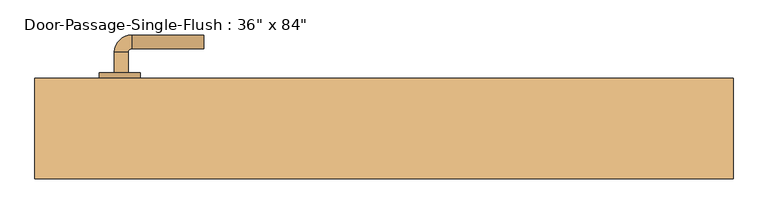
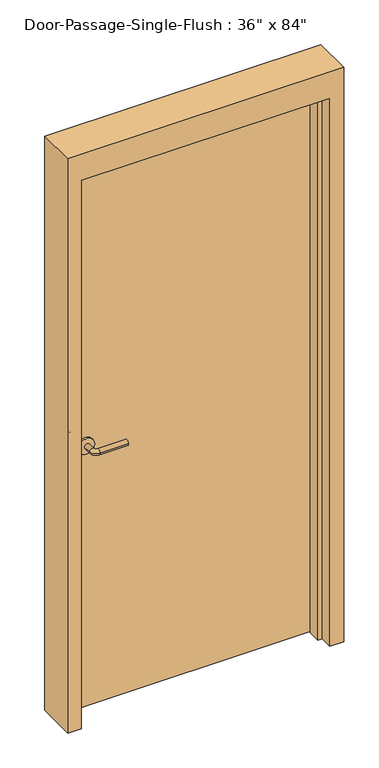
"""IFC4 building model written with IfcOpenShell, lengths in millimetres: door geometry."""

from ifc_helpers import new_model, si_unit, point, frame, frame_2d, origin, origin_with_axes, place, context, project, spatial, polyline, circle_curve, ellipse_curve, trimmed, segment, composite_curve, outline, extrude, faceted_brep, source, transform, mapped, element, save
from ifc_brep_helpers import plane_surface, cylinder_surface, revolved_surface, advanced_brep


def door_a255baf1(model_context):
    return source(origin(), model_context, "Body", "SolidModel", [
        advanced_brep(
        [(-392.190625, -1.65, 1016.0), (-372.190625, -1.65, 1016.0), (-372.190625, -31.65, 1016.0), (-392.190625, -31.65, 1016.0), (-367.190625, -36.65, 1016.0), (-367.190625, -56.65, 1016.0), (-262.190625, -56.65, 1016.0), (-262.190625, -36.65, 1016.0)],
        [
            (0, 1, circle_curve(frame((-382.190625, -1.65, 1016.0), z_axis=(0.0, 1.0, 0.0), x_axis=(1.0, 0.0, 0.0)), 10.0)),
            (1, 0, circle_curve(frame((-382.190625, -1.65, 1016.0), z_axis=(0.0, 1.0, 0.0), x_axis=(1.0, 0.0, 0.0)), 10.0)),
            (1, 2),
            (2, 3, circle_curve(frame((-382.190625, -31.65, 1016.0), z_axis=(0.0, 1.0, 0.0), x_axis=(1.0, 0.0, 0.0)), 10.0)),
            (3, 0),
            (3, 2, circle_curve(frame((-382.190625, -31.65, 1016.0), z_axis=(0.0, 1.0, 0.0), x_axis=(1.0, 0.0, 0.0)), 10.0)),
            (4, 5, circle_curve(frame((-367.190625, -46.65, 1016.0), z_axis=(-1.0, 0.0, 0.0), x_axis=(0.0, 1.0, 0.0)), 10.0)),
            (5, 3, circle_curve(frame((-367.190625, -31.65, 1016.0), z_axis=(0.0, 0.0, -1.0), x_axis=(-1.0, 0.0, 0.0)), 25.0)),
            (2, 4, circle_curve(frame((-367.190625, -31.65, 1016.0), z_axis=(0.0, 0.0, 1.0), x_axis=(-1.0, 0.0, 0.0)), 5.0)),
            (5, 4, circle_curve(frame((-367.190625, -46.65, 1016.0), z_axis=(-1.0, 0.0, 0.0), x_axis=(0.0, 1.0, 0.0)), 10.0)),
            (6, 7, circle_curve(frame((-262.190625, -46.65, 1016.0), z_axis=(1.0, 0.0, 0.0), x_axis=(0.0, 1.0, 0.0)), 10.0)),
            (7, 6, circle_curve(frame((-262.190625, -46.65, 1016.0), z_axis=(1.0, 0.0, 0.0), x_axis=(0.0, 1.0, 0.0)), 10.0)),
            (4, 7),
            (6, 5),
        ],
        [
            plane_surface(frame((-382.190625, -1.65, 1016.0), z_axis=(0.0, 1.0, 0.0), x_axis=(0.0, 0.0, 1.0))),
            cylinder_surface(frame((-382.190625, -1.65, 1016.0), z_axis=(0.0, 1.0, 0.0), x_axis=(1.0, 0.0, 0.0)), 10.0),
            revolved_surface(trimmed(ellipse_curve(frame((-382.190625, -31.65, 1016.0), z_axis=(0.0, -1.0, 0.0), x_axis=(1.0, 0.0, 0.0)), 10.0, 10.0), [point((-392.190625, -31.65, 1016.0))], [point((-372.190625, -31.65, 1016.0))], True, "CARTESIAN"), (-367.190625, -31.65, 1016.0), (0.0, 0.0, -1.0)),
            revolved_surface(trimmed(ellipse_curve(frame((-382.190625, -31.65, 1016.0), z_axis=(0.0, -1.0, 0.0), x_axis=(1.0, 0.0, 0.0)), 10.0, 10.0), [point((-372.190625, -31.65, 1016.0))], [point((-392.190625, -31.65, 1016.0))], True, "CARTESIAN"), (-367.190625, -31.65, 1016.0), (0.0, 0.0, -1.0)),
            plane_surface(frame((-262.190625, -46.65, 1016.0), z_axis=(1.0, 0.0, 0.0), x_axis=(0.0, 0.0, 1.0))),
            cylinder_surface(frame((-367.190625, -46.65, 1016.0), z_axis=(-1.0, 0.0, 0.0), x_axis=(0.0, 1.0, 0.0)), 10.0),
        ],
        [
            (0, [[1, 2]]),
            (1, [[3, 4, 5, -2]]),
            (1, [[-5, 6, -3, -1]]),
            (2, [[7, 8, -4, 9]]),
            (3, [[10, -9, -6, -8]]),
            (4, [[11, 12]]),
            (5, [[13, -11, 14, -7]]),
            (5, [[-14, -12, -13, -10]]),
        ],
    ),
        extrude(outline(composite_curve([segment(trimmed(circle_curve(frame_2d((1016.0, -384.690625)), 30.0), [point((1016.0, -414.690625))], [point((1016.0, -354.690625))], False, "CARTESIAN"), True, "CONTINUOUS"), segment(trimmed(circle_curve(frame_2d((1016.0, -384.690625)), 30.0), [point((1016.0, -354.690625))], [point((1016.0, -414.690625))], False, "CARTESIAN"), True, "CONTINUOUS")], self_intersect=False)), frame((0.0, -1.65, 0.0), z_axis=(0.0, 1.0, 0.0), x_axis=(0.0, 0.0, 1.0)), (0.0, 0.0, 1.0), 8.0),
        advanced_brep(
        [(-392.190625, 58.8, 1016.0), (-372.190625, 58.8, 1016.0), (-392.190625, 88.8, 1016.0), (-372.190625, 88.8, 1016.0), (-367.190625, 93.8, 1016.0), (-367.190625, 113.8, 1016.0), (-262.190625, 113.8, 1016.0), (-262.190625, 93.8, 1016.0)],
        [
            (0, 1, circle_curve(frame((-382.190625, 58.8, 1016.0), z_axis=(0.0, -1.0, 0.0), x_axis=(1.0, 0.0, 0.0)), 10.0)),
            (1, 0, circle_curve(frame((-382.190625, 58.8, 1016.0), z_axis=(0.0, -1.0, 0.0), x_axis=(1.0, 0.0, 0.0)), 10.0)),
            (0, 2),
            (2, 3, circle_curve(frame((-382.190625, 88.8, 1016.0), z_axis=(0.0, -1.0, 0.0), x_axis=(1.0, 0.0, 0.0)), 10.0)),
            (3, 1),
            (3, 2, circle_curve(frame((-382.190625, 88.8, 1016.0), z_axis=(0.0, -1.0, 0.0), x_axis=(1.0, 0.0, 0.0)), 10.0)),
            (4, 3, circle_curve(frame((-367.190625, 88.8, 1016.0), z_axis=(0.0, 0.0, 1.0), x_axis=(-1.0, 0.0, 0.0)), 5.0)),
            (2, 5, circle_curve(frame((-367.190625, 88.8, 1016.0), z_axis=(0.0, 0.0, -1.0), x_axis=(-1.0, 0.0, 0.0)), 25.0)),
            (5, 4, circle_curve(frame((-367.190625, 103.8, 1016.0), z_axis=(-1.0, 0.0, 0.0), x_axis=(0.0, -1.0, 0.0)), 10.0)),
            (4, 5, circle_curve(frame((-367.190625, 103.8, 1016.0), z_axis=(-1.0, 0.0, 0.0), x_axis=(0.0, -1.0, 0.0)), 10.0)),
            (6, 7, circle_curve(frame((-262.190625, 103.8, 1016.0), z_axis=(1.0, 0.0, 0.0), x_axis=(0.0, -1.0, 0.0)), 10.0)),
            (7, 6, circle_curve(frame((-262.190625, 103.8, 1016.0), z_axis=(1.0, 0.0, 0.0), x_axis=(0.0, -1.0, 0.0)), 10.0)),
            (5, 6),
            (7, 4),
        ],
        [
            plane_surface(frame((-382.190625, 58.8, 1016.0), z_axis=(0.0, -1.0, 0.0), x_axis=(0.0, 0.0, 1.0))),
            cylinder_surface(frame((-382.190625, 58.8, 1016.0), z_axis=(0.0, -1.0, 0.0), x_axis=(1.0, 0.0, 0.0)), 10.0),
            revolved_surface(trimmed(ellipse_curve(frame((-382.190625, 88.8, 1016.0), z_axis=(0.0, -1.0, 0.0), x_axis=(1.0, 0.0, 0.0)), 10.0, 10.0), [point((-392.190625, 88.8, 1016.0))], [point((-372.190625, 88.8, 1016.0))], True, "CARTESIAN"), (-367.190625, 88.8, 1016.0), (0.0, 0.0, -1.0)),
            revolved_surface(trimmed(ellipse_curve(frame((-382.190625, 88.8, 1016.0), z_axis=(0.0, -1.0, 0.0), x_axis=(1.0, 0.0, 0.0)), 10.0, 10.0), [point((-372.190625, 88.8, 1016.0))], [point((-392.190625, 88.8, 1016.0))], True, "CARTESIAN"), (-367.190625, 88.8, 1016.0), (0.0, 0.0, -1.0)),
            plane_surface(frame((-262.190625, 103.8, 1016.0), z_axis=(1.0, 0.0, 0.0), x_axis=(0.0, 0.0, 1.0))),
            cylinder_surface(frame((-367.190625, 103.8, 1016.0), z_axis=(-1.0, 0.0, 0.0), x_axis=(0.0, -1.0, 0.0)), 10.0),
        ],
        [
            (0, [[1, 2]]),
            (1, [[-1, 3, 4, 5]]),
            (1, [[-2, -5, 6, -3]]),
            (2, [[7, -4, 8, 9]]),
            (3, [[-8, -6, -7, 10]]),
            (4, [[11, 12]]),
            (5, [[-9, 13, -12, 14]]),
            (5, [[-10, -14, -11, -13]]),
        ],
    ),
        extrude(outline(composite_curve([segment(trimmed(circle_curve(frame_2d((1016.0, -384.690625)), 30.0), [point((1016.0, -414.690625))], [point((1016.0, -354.690625))], False, "CARTESIAN"), True, "CONTINUOUS"), segment(trimmed(circle_curve(frame_2d((1016.0, -384.690625)), 30.0), [point((1016.0, -354.690625))], [point((1016.0, -414.690625))], False, "CARTESIAN"), True, "CONTINUOUS")], self_intersect=False)), frame((0.0, 50.8, 0.0), z_axis=(0.0, 1.0, 0.0), x_axis=(0.0, 0.0, 1.0)), (0.0, 0.0, 1.0), 8.0),
        faceted_brep([(457.2, 1.5875, 0.0), (457.2, 50.8, 0.0), (508.0, 50.8, 0.0), (508.0, -95.25, 0.0), (457.2, -95.25, 0.0), (457.2, -46.0375, 0.0), (441.325, -46.0375, 0.0), (441.325, 1.5875, 0.0), (457.2, 1.5875, 2133.6), (457.2, 50.8, 2133.6), (-457.2, 50.8, 2133.6), (-457.2, 50.8, 0.0), (-508.0, 50.8, 0.0), (-508.0, 50.8, 2235.2), (508.0, 50.8, 2235.2), (508.0, -95.25, 2235.2), (-508.0, -95.25, 2235.2), (-508.0, -95.25, 0.0), (-457.2, -95.25, 0.0), (-457.2, -95.25, 2133.6), (457.2, -95.25, 2133.6), (457.2, -46.0375, 2133.6), (-457.2, -46.0375, 2133.6), (-457.2, -46.0375, 0.0), (-441.325, -46.0375, 0.0), (-441.325, -46.0375, 2117.725), (441.325, -46.0375, 2117.725), (441.325, 1.5875, 2117.725), (-441.325, 1.5875, 2117.725), (-441.325, 1.5875, 0.0), (-457.2, 1.5875, 0.0), (-457.2, 1.5875, 2133.6)], [[[0, 1, 2, 3, 4, 5, 6, 7]], [[1, 0, 8, 9]], [[2, 1, 9, 10, 11, 12, 13, 14]], [[3, 2, 14, 15]], [[4, 3, 15, 16, 17, 18, 19, 20]], [[5, 4, 20, 21]], [[6, 5, 21, 22, 23, 24, 25, 26]], [[7, 6, 26, 27]], [[0, 7, 27, 28, 29, 30, 31, 8]], [[9, 8, 31, 10]], [[20, 19, 22, 21]], [[26, 25, 28, 27]], [[12, 11, 30, 29, 24, 23, 18, 17]], [[11, 10, 31, 30]], [[13, 12, 17, 16]], [[19, 18, 23, 22]], [[25, 24, 29, 28]], [[15, 14, 13, 16]]]),
        extrude(outline(polyline([(457.2, 6.35), (-457.2, 6.35), (-457.2, 50.8), (457.2, 50.8), (457.2, 6.35)])), origin_with_axes(), (0.0, 0.0, 1.0), 2133.6),
    ])


if __name__ == "__main__":
    model = new_model("IFC4")
    model_context = context("Model", 3, world=origin())
    ifc_project = project(units=[si_unit("LENGTHUNIT", "METRE", prefix="MILLI")], contexts=[model_context])
    site = spatial("IfcSite", under=ifc_project)
    building = spatial("IfcBuilding", under=site)
    placement = place(None, origin())
    door_shape = door_a255baf1(model_context)
    element("IfcDoor", 1, ObjectType="Door-Passage-Single-Flush : 36\" x 84\"", at=placement, inside=building, context=model_context, shape_type="MappedRepresentation", body=[
        mapped(door_shape, transform((0.0, 0.0, 0.0), x_axis=(1.0, 0.0, 0.0), y_axis=(0.0, 1.0, 0.0), z_axis=(0.0, 0.0, 1.0))),
    ])
    save(model, "model.ifc")

# Revit data of these elements
# Type "Door-Passage-Single-Flush : 36\" x 84\""
#   Type Mark = "35"
#   Assembly Code = "B2030200"
#   Analytic Construction = "Wooden"
#   Thickness = 0' - 1 3/4"
#   Thermal Resistance (R) = 2.5876 (h·ft²·°F)/BTU
#   Swing Angle [instance default] = 90.00°
#   Strike Height = 3' - 4"
#   Rough Width [instance default] = 3' - 4"
#   Rough Height [instance default] = 7' - 4"
#   MF Opening Height [instance default] = 0' - 4"
#   MF Opening Width [instance default] = 0' - 4"
#   Inset Calculate [instance default] = 0' - 4"
#   Masonry Inset [instance default] = 0' - 1"
#   Height = 7' - 0"
#   Width = 3' - 0"
#   Heat Transfer Coefficient (U) = 0.3865 BTU/(h·ft²·°F)
#   Masonry Frame Depth = 0' - 5 3/4"
#   Masonry Frame [instance default] = yes
#   Function = 1
#   Dry Wall Frame [instance default] = no
#   Panel Material = Wood - Birch
#   Frame Material = Metal - Paint Finish - Grey
#   Door Handle Material = Aluminum
#   Visual Light Transmittance = 0
#   Solar Heat Gain Coefficient = 0
#   Wall Closure = (empty or 0)
# Element 1 (IfcDoor, "Door-Passage-Single-Flush : 36\" x 84\"")
#   Materials on its faces: "Aluminum", "Metal - Paint Finish - Grey", "Wood - Birch"
# Materials
#   "Wood - Birch": class "Wood", colour RGB 166 116 52, transparency 0, Cost = 0
#   "Metal - Paint Finish - Grey": class "Paint", colour RGB 104 104 104, transparency 0, Cost = 0
#   "Aluminum": class "Metal", colour RGB 247 247 247, transparency 0, Description = "Aluminum 6061", Cost = 0
